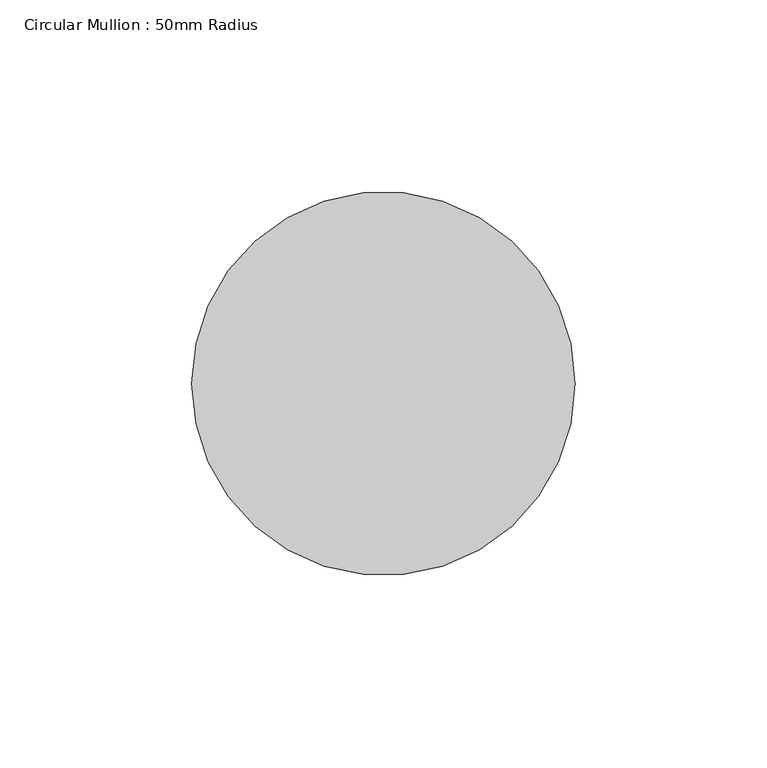
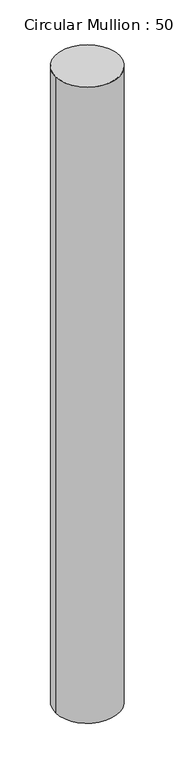
"""IFC4 building model written with IfcOpenShell, lengths in millimetres: member geometry, Circular Mullion : 50mm Radius."""

from ifc_helpers import new_model, si_unit, point, frame, origin, origin_2d, place, context, project, spatial, circle_curve, trimmed, segment, composite_curve, outline, extrude, source, transform, mapped, element, save


def circular_mullion_50mm_radius_88f33baa(model_context):
    return source(origin(), model_context, "Body", "SweptSolid", [
        extrude(outline(composite_curve([segment(trimmed(circle_curve(origin_2d(), 50.0), [point((50.0, 0.0))], [point((-50.0, 0.0))], False, "CARTESIAN"), True, "CONTINUOUS"), segment(trimmed(circle_curve(origin_2d(), 50.0), [point((-50.0, 0.0))], [point((50.0, 0.0))], False, "CARTESIAN"), True, "CONTINUOUS")], self_intersect=False)), frame((0.0, 0.0, -1049.2326044), z_axis=(0.0, 0.0, 1.0), x_axis=(1.0, 0.0, 0.0)), (0.0, 0.0, 1.0), 1049.2326044),
    ])


if __name__ == "__main__":
    model = new_model("IFC4")
    model_context = context("Model", 3, world=origin())
    ifc_project = project(units=[si_unit("LENGTHUNIT", "METRE", prefix="MILLI")], contexts=[model_context])
    site = spatial("IfcSite", under=ifc_project)
    building = spatial("IfcBuilding", under=site)
    placement = place(None, origin())
    circular_mullion_50mm_radius_shape = circular_mullion_50mm_radius_88f33baa(model_context)
    element("IfcMember", 1, ObjectType="Circular Mullion : 50mm Radius", at=placement, inside=building, context=model_context, shape_type="MappedRepresentation", body=[
        mapped(circular_mullion_50mm_radius_shape, transform((0.0, 0.0, 0.0), x_axis=(1.0, 0.0, 0.0), y_axis=(0.0, 1.0, 0.0), z_axis=(0.0, 0.0, 1.0))),
    ])
    save(model, "model.ifc")

# Revit data of these elements
# Type "Circular Mullion : 50mm Radius"
#   built-in parameter 1007350 = 0.164042 (stored number, unit not read)
# Element 1 (IfcMember, "Circular Mullion : 50mm Radius")
#   Materials on its faces: "Aluminium"
# Materials
#   "Aluminium": class "Metal", colour RGB 247 247 247, transparency 0, Description = "Aluminium 6061", Cost = 0
